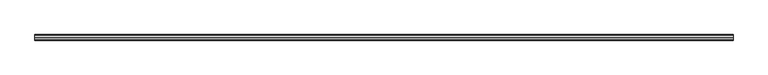
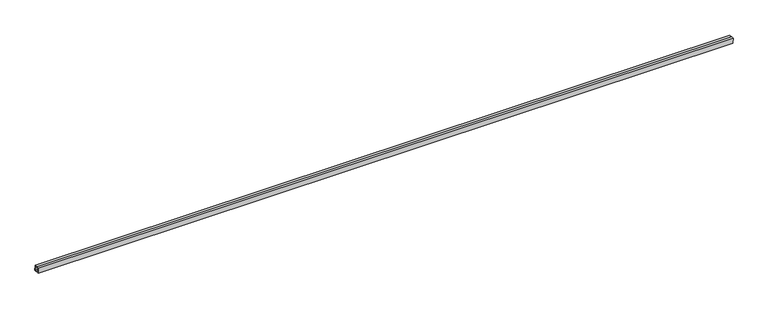
"""IFC4 building model written with IfcOpenShell, lengths in millimetres: proxy geometry, Inner panel:Inner panel:1:Inner panel:1 : Inner panel:Inner panel:300324:2:Inner panel:1:Inner panel:1 : Inner panel:Inner panel:300324:2 : Inner panel:Inner panel:1:Inner panel:1 : Inner panel:Inner panel:300324:300043:26 : Inner panel:Inner panel:1:Inner panel:1 : Inner panel:Inner panel:300324:2:Inner panel:1:Inner panel:1 : Inner panel:Inner panel:300324:2 : Inner panel:Inner panel:1:Inner panel:1 : Inner panel:Inner panel:300324:300043:308120."""

import ifcopenshell
import ifcopenshell.guid

model = None  # the IFC model being written
_history = None  # IfcOwnerHistory: only IFC2X3 demands one
_inside = {}  # id of a spatial element -> (the spatial element, [elements in it])
_under = {}  # id of a project, library or spatial element -> (it, [spatial elements below it])
_declared = {}  # id of a project -> (the project, [libraries it declares])
_typed = {}  # id of a type object -> (the type object, [elements of that type])
_made_of = {}  # id of a material, layer set ... -> (it, [elements and type objects made of it])


def new_model(schema):
    """Start an empty IFC model of exactly this schema.

    Asked for "IFC4X3", IfcOpenShell would pick the latest addendum, in which some entities
    have other attributes; the version numbers below select the first issue.
    IFC2X3 requires an IfcOwnerHistory on every rooted entity: one is made here for all.
    """
    global model, _history
    if schema == "IFC4X3":
        model = ifcopenshell.file(schema_version=(4, 3, 0, 0))
    else:
        model = ifcopenshell.file(schema=schema)
    _inside.clear()
    _under.clear()
    _declared.clear()
    _typed.clear()
    _made_of.clear()
    _history = None
    if model.schema == "IFC2X3":
        org = make("IfcOrganization", Name="unknown")
        user = make(
            "IfcPersonAndOrganization",
            ThePerson=make("IfcPerson", FamilyName="unknown"),
            TheOrganization=org,
        )
        app = make(
            "IfcApplication",
            ApplicationDeveloper=org,
            Version="unknown",
            ApplicationFullName="unknown",
            ApplicationIdentifier="unknown",
        )
        _history = make(
            "IfcOwnerHistory",
            OwningUser=user,
            OwningApplication=app,
            ChangeAction="ADDED",
            CreationDate=0,
        )
    return model


def make(cls, **values):
    """One entity of the class cls with the attributes given. An attribute that is None is left unset."""
    return model.create_entity(
        cls, **{name: value for name, value in values.items() if value is not None}
    )


def rooted(cls, **values):
    """An entity with a GlobalId (a new one), such as an element, a storey or a relation."""
    return make(cls, GlobalId=ifcopenshell.guid.new(), OwnerHistory=_history, **values)


def si_unit(unit_type, name, prefix=None):
    """IfcSIUnit, for example si_unit("LENGTHUNIT", "METRE", prefix="MILLI")."""
    return make("IfcSIUnit", UnitType=unit_type, Prefix=prefix, Name=name)


def assignment(units):
    """IfcUnitAssignment: the units of a project."""
    return None if units is None else make("IfcUnitAssignment", Units=units)


def point(xyz):
    """IfcCartesianPoint."""
    return None if xyz is None else make("IfcCartesianPoint", Coordinates=xyz)


def direction(xyz):
    """IfcDirection."""
    return None if xyz is None else make("IfcDirection", DirectionRatios=xyz)


def frame(location, z_axis=None, x_axis=None):
    """IfcAxis2Placement3D, a coordinate frame: its origin and axes. An axis left out is left unset."""
    return make(
        "IfcAxis2Placement3D",
        Location=point(location),
        Axis=direction(z_axis),
        RefDirection=direction(x_axis),
    )


def origin():
    """The frame at (0, 0, 0) with its axes left unset."""
    return frame((0.0, 0.0, 0.0))


def place(relative_to, where):
    """IfcLocalPlacement: puts the frame where relative to a parent placement (None: the world)."""
    return make(
        "IfcLocalPlacement", PlacementRelTo=relative_to, RelativePlacement=where
    )


def context(
    kind, dimensions, precision=None, world=None, true_north=None, identifier=None
):
    """IfcGeometricRepresentationContext, for example the 3D "Model" context."""
    return make(
        "IfcGeometricRepresentationContext",
        ContextIdentifier=identifier,
        ContextType=kind,
        CoordinateSpaceDimension=dimensions,
        Precision=precision,
        WorldCoordinateSystem=world,
        TrueNorth=true_north,
    )


def project(units=None, contexts=None):
    """IfcProject with its units and contexts."""
    return rooted(
        "IfcProject",
        Name="project",
        RepresentationContexts=contexts,
        UnitsInContext=assignment(units),
    )


def spatial(cls, under=None, at=None, **own):
    """A site, building, storey or space (cls), placed at a placement, below another one or the project."""
    s = rooted(cls, ObjectPlacement=at, **own)
    if under is not None:
        _under.setdefault(under.id(), (under, []))[1].append(s)
    return s


def polyline(points):
    """IfcPolyline through the points."""
    return make("IfcPolyline", Points=[point(p) for p in points])


def outline(outer, holes=None, kind="AREA"):
    """IfcArbitraryClosedProfileDef: a profile drawn as a closed curve; with holes, ...WithVoids."""
    if holes is None:
        return make("IfcArbitraryClosedProfileDef", ProfileType=kind, OuterCurve=outer)
    return make(
        "IfcArbitraryProfileDefWithVoids",
        ProfileType=kind,
        OuterCurve=outer,
        InnerCurves=holes,
    )


def extrude(swept, where, along, depth):
    """IfcExtrudedAreaSolid: the profile swept, set in the frame where, extruded along a direction by depth."""
    return make(
        "IfcExtrudedAreaSolid",
        SweptArea=swept,
        Position=where,
        ExtrudedDirection=direction(along),
        Depth=depth,
    )


def shape(context_of_items, identifier, shape_type, items):
    """IfcShapeRepresentation: the items that make up one representation, for example the "Body"."""
    return make(
        "IfcShapeRepresentation",
        ContextOfItems=context_of_items,
        RepresentationIdentifier=identifier,
        RepresentationType=shape_type,
        Items=items,
    )


def source(mapping_origin, context_of_items, identifier, shape_type, items):
    """IfcRepresentationMap: a shape defined once, which mapped items show again and again."""
    return make(
        "IfcRepresentationMap",
        MappingOrigin=mapping_origin,
        MappedRepresentation=shape(context_of_items, identifier, shape_type, items),
    )


def transform(
    local_origin,
    x_axis=None,
    y_axis=None,
    z_axis=None,
    scale=None,
    scale2=None,
    scale3=None,
    uniform=True,
):
    """IfcCartesianTransformationOperator3D, or its non-uniform kind. x_axis, y_axis, z_axis: its Axis1, 2, 3."""
    if uniform:
        return make(
            "IfcCartesianTransformationOperator3D",
            Axis1=direction(x_axis),
            Axis2=direction(y_axis),
            LocalOrigin=point(local_origin),
            Scale=scale,
            Axis3=direction(z_axis),
        )
    return make(
        "IfcCartesianTransformationOperator3DnonUniform",
        Axis1=direction(x_axis),
        Axis2=direction(y_axis),
        LocalOrigin=point(local_origin),
        Scale=scale,
        Axis3=direction(z_axis),
        Scale2=scale2,
        Scale3=scale3,
    )


def mapped(mapping_source, mapping_target):
    """IfcMappedItem: shows the shape of a source again, moved by a transform."""
    return make(
        "IfcMappedItem", MappingSource=mapping_source, MappingTarget=mapping_target
    )


def made_of(thing, what):
    """Note that an element or type object is made of a material, layer set ...; save() writes the relation."""
    if what is not None:
        _made_of.setdefault(what.id(), (what, []))[1].append(thing)
    return thing


def element(
    cls,
    number,
    at=None,
    inside=None,
    cuts=None,
    type_object=None,
    material=None,
    context=None,
    identifier="Body",
    shape_type=None,
    held_by="IfcProductDefinitionShape",
    body=None,
    shapes=None,
    **own,
):
    """One element of the class cls, such as IfcWall. Its Tag is "e" and its number.

    at: its placement. inside: the storey or other place that contains it. cuts: it is an
    opening in that element (IfcRelVoidsElement). A single representation is given by context,
    identifier, shape_type and body (its items); several are given by shapes. held_by: the class
    of the entity that holds the representations. save() writes the other relations.
    """
    e = rooted(cls, Tag="e%d" % number, ObjectPlacement=at, **own)
    if body is not None:
        shapes = [shape(context, identifier, shape_type, body)]
    if shapes is not None:
        e.Representation = make(held_by, Representations=shapes)
    if inside is not None:
        _inside.setdefault(inside.id(), (inside, []))[1].append(e)
    if cuts is not None:
        rooted(
            "IfcRelVoidsElement", RelatingBuildingElement=cuts, RelatedOpeningElement=e
        )
    if type_object is not None:
        _typed.setdefault(type_object.id(), (type_object, []))[1].append(e)
    return made_of(e, material)


def aggregate(whole, parts):
    """IfcRelAggregates: a whole, such as a stair, and the parts it consists of."""
    return rooted("IfcRelAggregates", RelatingObject=whole, RelatedObjects=parts)


def save(model, path):
    """Write the relations noted so far, then the file.

    IfcRelAggregates (storeys below a building ...), IfcRelContainedInSpatialStructure (elements
    in a storey), IfcRelDefinesByType, IfcRelAssociatesMaterial and IfcRelDeclares: one each for
    every whole, place, type object, material and project.
    """
    for whole, parts in _under.values():
        aggregate(whole, parts)
    for where, things in _inside.values():
        rooted(
            "IfcRelContainedInSpatialStructure",
            RelatedElements=things,
            RelatingStructure=where,
        )
    for kind, things in _typed.values():
        rooted("IfcRelDefinesByType", RelatedObjects=things, RelatingType=kind)
    for what, things in _made_of.values():
        rooted("IfcRelAssociatesMaterial", RelatedObjects=things, RelatingMaterial=what)
    for by, libraries in _declared.values():
        rooted("IfcRelDeclares", RelatingContext=by, RelatedDefinitions=libraries)
    model.write(path)


def generic_models_7b1811bf(model_context):
    return source(origin(), model_context, "Body", "SweptSolid", [
        extrude(outline(polyline([(-569791.292732, 8736.8354816), (-569773.0523088, 8737.5954993), (-569771.4661851, 8699.5285292), (-569809.5331552, 8697.9424054), (-569811.1192789, 8736.0093755), (-569792.8788557, 8736.7693931), (-569792.779723, 8734.3902075), (-569808.6409605, 8733.7293226), (-569807.2531023, 8700.4207238), (-569773.9445034, 8701.8085821), (-569775.3323617, 8735.1171809), (-569791.1935993, 8734.456296), (-569791.292732, 8736.8354816)])), frame((588245.3367242, 0.0, 0.0), z_axis=(1.0, 0.0, 0.0), x_axis=(0.0, 1.0, 0.0)), (0.0, 0.0, 1.0), 4876.8),
    ])


if __name__ == "__main__":
    model = new_model("IFC4")
    model_context = context("Model", 3, world=origin())
    ifc_project = project(units=[si_unit("LENGTHUNIT", "METRE", prefix="MILLI")], contexts=[model_context])
    site = spatial("IfcSite", under=ifc_project)
    building = spatial("IfcBuilding", under=site)
    placement = place(None, origin())
    generic_models_shape = generic_models_7b1811bf(model_context)
    element("IfcBuildingElementProxy", 1, Name="Inner panel:Inner panel:1:Inner panel:1 : Inner panel:Inner panel:300324:2:Inner panel:1:Inner panel:1 : Inner panel:Inner panel:300324:2 : Inner panel:Inner panel:1:Inner panel:1 : Inner panel:Inner panel:300324:300043:26 : Inner panel:Inner panel:1:Inner panel:1 : Inner panel:Inner panel:300324:2:Inner panel:1:Inner panel:1 : Inner panel:Inner panel:300324:2 : Inner panel:Inner panel:1:Inner panel:1 : Inner panel:Inner panel:300324:300043:308120", ObjectType="Inner panel:Inner panel:1:Inner panel:1 : Inner panel:Inner panel:300324:2:Inner panel:1:Inner panel:1 : Inner panel:Inner panel:300324:2 : Inner panel:Inner panel:1:Inner panel:1 : Inner panel:Inner panel:300324:300043:26 : Inner panel:Inner panel:1:Inner panel:1 : Inner panel:Inner panel:300324:2:Inner panel:1:Inner panel:1 : Inner panel:Inner panel:300324:2 : Inner panel:Inner panel:1:Inner panel:1 : Inner panel:Inner panel:300324:300043:308120", at=placement, inside=building, context=model_context, shape_type="MappedRepresentation", body=[
        mapped(generic_models_shape, transform((0.0, 0.0, 0.0), x_axis=(1.0, 0.0, 0.0), y_axis=(0.0, 1.0, 0.0), z_axis=(0.0, 0.0, 1.0))),
    ])
    save(model, "model.ifc")

# Revit data of these elements
# Type "Inner panel:Inner panel:1:Inner panel:1 : Inner panel:Inner panel:300324:2:Inner panel:1:Inner panel:1 : Inner panel:Inner panel:300324:2 : Inner panel:Inner panel:1:Inner panel:1 : Inner panel:Inner panel:300324:300043:26 : Inner panel:Inner panel:1:Inner panel:1 : Inner panel:Inner panel:300324:2:Inner panel:1:Inner panel:1 : Inner panel:Inner panel:300324:2 : Inner panel:Inner panel:1:Inner panel:1 : Inner panel:Inner panel:300324:300043:308120"
#   NameOverride = "Inner panel:Inner panel:1:Inner panel:1 : Inner panel:Inner panel:300324:2:Inner panel:1:Inner panel:1 : Inner panel:Inner panel:300324:2 : Inner panel:Inner panel:1:Inner panel:1 : Inner panel:Inner panel:300324:300043:308120"
#   ObjectTypeOverride = "Inner panel:1:Inner panel:1 : Inner panel:Inner panel:300324:2 : Inner panel:Inner panel:1:Inner panel:1 : Inner panel:Inner panel:300324:300043"
#   Reference = "Inner panel"
#   Tag = "308120"
# Element 1 (IfcBuildingElementProxy, "Inner panel:Inner panel:1:Inner panel:1 : Inner panel:Inner panel:300324:2:Inner panel:1:Inner panel:1 : Inner panel:Inner panel:300324:2 : Inner panel:Inner panel:1:Inner panel:1 : Inner panel:Inner panel:300324:300043:26 : Inner panel:Inner panel:1:Inner panel:1 : Inner panel:Inner panel:300324:2:Inner panel:1:Inner panel:1 : Inner panel:Inner panel:300324:2 : Inner panel:Inner panel:1:Inner panel:1 : Inner panel:Inner panel:300324:300043:308120")
#   Materials on its faces: "1 1/2\" X 1 1/2\" SPLIT-SEAM SQUARE TUBING (~24\" CANTILEVER FROM C.L. OF GLULAM)"
# Materials
#   "1 1/2\" X 1 1/2\" SPLIT-SEAM SQUARE TUBING (~24\" CANTILEVER FROM C.L. OF GLULAM)": class "Unassigned", colour RGB 202 201 200, transparency 0, Cost = 0
